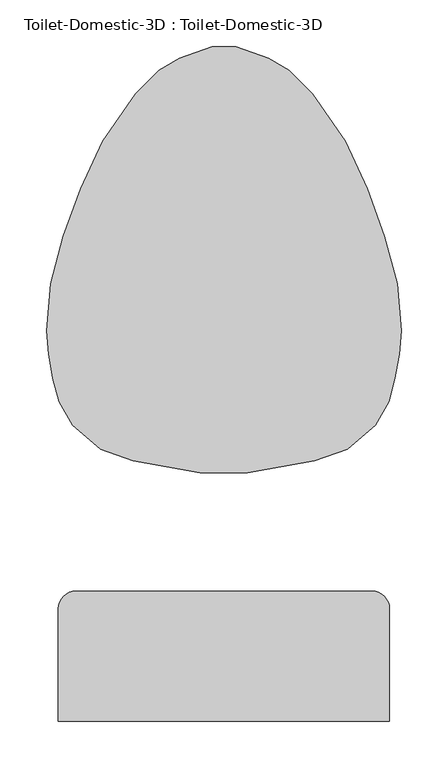
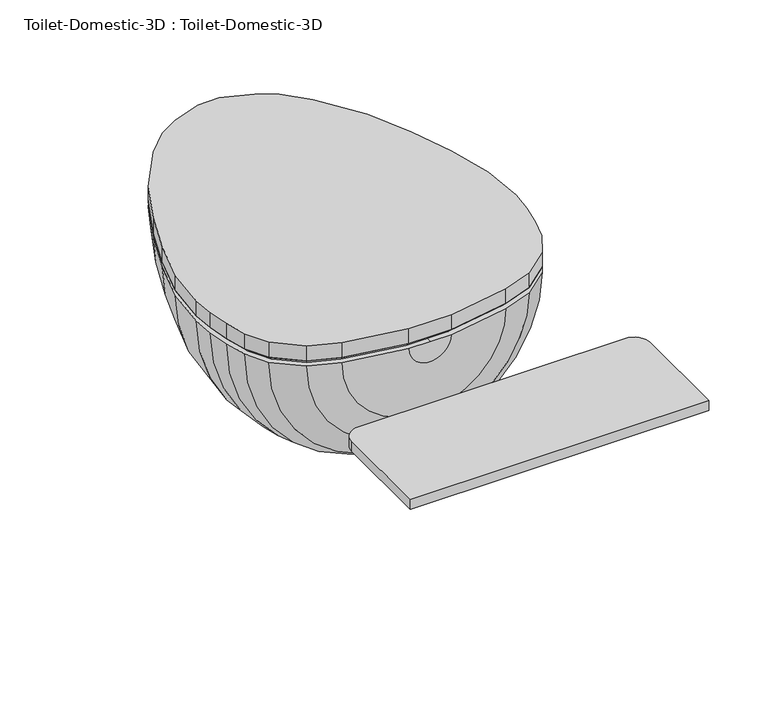
"""IFC4 building model written with IfcOpenShell, lengths in millimetres: flow terminal geometry, Toilet-Domestic-3D : Toilet-Domestic-3D."""

import ifcopenshell
import ifcopenshell.guid

model = None  # the IFC model being written
_history = None  # IfcOwnerHistory: only IFC2X3 demands one
_inside = {}  # id of a spatial element -> (the spatial element, [elements in it])
_under = {}  # id of a project, library or spatial element -> (it, [spatial elements below it])
_declared = {}  # id of a project -> (the project, [libraries it declares])
_typed = {}  # id of a type object -> (the type object, [elements of that type])
_made_of = {}  # id of a material, layer set ... -> (it, [elements and type objects made of it])


def new_model(schema):
    """Start an empty IFC model of exactly this schema.

    Asked for "IFC4X3", IfcOpenShell would pick the latest addendum, in which some entities
    have other attributes; the version numbers below select the first issue.
    IFC2X3 requires an IfcOwnerHistory on every rooted entity: one is made here for all.
    """
    global model, _history
    if schema == "IFC4X3":
        model = ifcopenshell.file(schema_version=(4, 3, 0, 0))
    else:
        model = ifcopenshell.file(schema=schema)
    _inside.clear()
    _under.clear()
    _declared.clear()
    _typed.clear()
    _made_of.clear()
    _history = None
    if model.schema == "IFC2X3":
        org = make("IfcOrganization", Name="unknown")
        user = make(
            "IfcPersonAndOrganization",
            ThePerson=make("IfcPerson", FamilyName="unknown"),
            TheOrganization=org,
        )
        app = make(
            "IfcApplication",
            ApplicationDeveloper=org,
            Version="unknown",
            ApplicationFullName="unknown",
            ApplicationIdentifier="unknown",
        )
        _history = make(
            "IfcOwnerHistory",
            OwningUser=user,
            OwningApplication=app,
            ChangeAction="ADDED",
            CreationDate=0,
        )
    return model


def make(cls, **values):
    """One entity of the class cls with the attributes given. An attribute that is None is left unset."""
    return model.create_entity(
        cls, **{name: value for name, value in values.items() if value is not None}
    )


def rooted(cls, **values):
    """An entity with a GlobalId (a new one), such as an element, a storey or a relation."""
    return make(cls, GlobalId=ifcopenshell.guid.new(), OwnerHistory=_history, **values)


def si_unit(unit_type, name, prefix=None):
    """IfcSIUnit, for example si_unit("LENGTHUNIT", "METRE", prefix="MILLI")."""
    return make("IfcSIUnit", UnitType=unit_type, Prefix=prefix, Name=name)


def assignment(units):
    """IfcUnitAssignment: the units of a project."""
    return None if units is None else make("IfcUnitAssignment", Units=units)


def point(xyz):
    """IfcCartesianPoint."""
    return None if xyz is None else make("IfcCartesianPoint", Coordinates=xyz)


def direction(xyz):
    """IfcDirection."""
    return None if xyz is None else make("IfcDirection", DirectionRatios=xyz)


def frame(location, z_axis=None, x_axis=None):
    """IfcAxis2Placement3D, a coordinate frame: its origin and axes. An axis left out is left unset."""
    return make(
        "IfcAxis2Placement3D",
        Location=point(location),
        Axis=direction(z_axis),
        RefDirection=direction(x_axis),
    )


def frame_2d(location, x_axis=None):
    """IfcAxis2Placement2D, a coordinate frame in the plane: its origin and x axis."""
    return make(
        "IfcAxis2Placement2D", Location=point(location), RefDirection=direction(x_axis)
    )


def origin():
    """The frame at (0, 0, 0) with its axes left unset."""
    return frame((0.0, 0.0, 0.0))


def place(relative_to, where):
    """IfcLocalPlacement: puts the frame where relative to a parent placement (None: the world)."""
    return make(
        "IfcLocalPlacement", PlacementRelTo=relative_to, RelativePlacement=where
    )


def context(
    kind, dimensions, precision=None, world=None, true_north=None, identifier=None
):
    """IfcGeometricRepresentationContext, for example the 3D "Model" context."""
    return make(
        "IfcGeometricRepresentationContext",
        ContextIdentifier=identifier,
        ContextType=kind,
        CoordinateSpaceDimension=dimensions,
        Precision=precision,
        WorldCoordinateSystem=world,
        TrueNorth=true_north,
    )


def project(units=None, contexts=None):
    """IfcProject with its units and contexts."""
    return rooted(
        "IfcProject",
        Name="project",
        RepresentationContexts=contexts,
        UnitsInContext=assignment(units),
    )


def spatial(cls, under=None, at=None, **own):
    """A site, building, storey or space (cls), placed at a placement, below another one or the project."""
    s = rooted(cls, ObjectPlacement=at, **own)
    if under is not None:
        _under.setdefault(under.id(), (under, []))[1].append(s)
    return s


def polyline(points):
    """IfcPolyline through the points."""
    return make("IfcPolyline", Points=[point(p) for p in points])


def circle_curve(where, radius):
    """IfcCircle in the frame where."""
    return make("IfcCircle", Position=where, Radius=radius)


def trimmed(basis, trim1, trim2, sense, master):
    """IfcTrimmedCurve: the piece of a basis curve between two trims."""
    return make(
        "IfcTrimmedCurve",
        BasisCurve=basis,
        Trim1=trim1,
        Trim2=trim2,
        SenseAgreement=sense,
        MasterRepresentation=master,
    )


def segment(curve, same_sense, transition):
    """IfcCompositeCurveSegment."""
    return make(
        "IfcCompositeCurveSegment",
        Transition=transition,
        SameSense=same_sense,
        ParentCurve=curve,
    )


def composite_curve(segments, self_intersect=None):
    """IfcCompositeCurve: segments joined end to end."""
    return make("IfcCompositeCurve", Segments=segments, SelfIntersect=self_intersect)


def outline(outer, holes=None, kind="AREA"):
    """IfcArbitraryClosedProfileDef: a profile drawn as a closed curve; with holes, ...WithVoids."""
    if holes is None:
        return make("IfcArbitraryClosedProfileDef", ProfileType=kind, OuterCurve=outer)
    return make(
        "IfcArbitraryProfileDefWithVoids",
        ProfileType=kind,
        OuterCurve=outer,
        InnerCurves=holes,
    )


def extrude(swept, where, along, depth):
    """IfcExtrudedAreaSolid: the profile swept, set in the frame where, extruded along a direction by depth."""
    return make(
        "IfcExtrudedAreaSolid",
        SweptArea=swept,
        Position=where,
        ExtrudedDirection=direction(along),
        Depth=depth,
    )


def faces_of(points, faces, orient=None, outer=None):
    """IfcFace entities. A face is a list of loops; a loop is a list of indices into points, from 0.

    orient and outer hold one flag for each loop. By default every Orientation is true, the
    first loop of a face is its IfcFaceOuterBound and the others are IfcFaceBound.
    """
    made = []
    for i, loops in enumerate(faces):
        bounds = []
        for j, loop in enumerate(loops):
            is_outer = j == 0 if outer is None else outer[i][j]
            bounds.append(
                make(
                    "IfcFaceOuterBound" if is_outer else "IfcFaceBound",
                    Bound=make("IfcPolyLoop", Polygon=[points[k] for k in loop]),
                    Orientation=True if orient is None else orient[i][j],
                )
            )
        made.append(make("IfcFace", Bounds=bounds))
    return made


def faceted_brep(points, faces, orient=None, outer=None, voids=None):
    """IfcFacetedBrep: a solid bounded by flat faces; with voids (closed shells), ...WithVoids."""
    shared = [point(p) for p in points]
    hull = make("IfcClosedShell", CfsFaces=faces_of(shared, faces, orient, outer))
    if voids is None:
        return make("IfcFacetedBrep", Outer=hull)
    return make(
        "IfcFacetedBrepWithVoids",
        Outer=hull,
        Voids=[
            make(cls, CfsFaces=faces_of(shared, fs, o, b)) for cls, fs, o, b in voids
        ],
    )


def shape(context_of_items, identifier, shape_type, items):
    """IfcShapeRepresentation: the items that make up one representation, for example the "Body"."""
    return make(
        "IfcShapeRepresentation",
        ContextOfItems=context_of_items,
        RepresentationIdentifier=identifier,
        RepresentationType=shape_type,
        Items=items,
    )


def source(mapping_origin, context_of_items, identifier, shape_type, items):
    """IfcRepresentationMap: a shape defined once, which mapped items show again and again."""
    return make(
        "IfcRepresentationMap",
        MappingOrigin=mapping_origin,
        MappedRepresentation=shape(context_of_items, identifier, shape_type, items),
    )


def transform(
    local_origin,
    x_axis=None,
    y_axis=None,
    z_axis=None,
    scale=None,
    scale2=None,
    scale3=None,
    uniform=True,
):
    """IfcCartesianTransformationOperator3D, or its non-uniform kind. x_axis, y_axis, z_axis: its Axis1, 2, 3."""
    if uniform:
        return make(
            "IfcCartesianTransformationOperator3D",
            Axis1=direction(x_axis),
            Axis2=direction(y_axis),
            LocalOrigin=point(local_origin),
            Scale=scale,
            Axis3=direction(z_axis),
        )
    return make(
        "IfcCartesianTransformationOperator3DnonUniform",
        Axis1=direction(x_axis),
        Axis2=direction(y_axis),
        LocalOrigin=point(local_origin),
        Scale=scale,
        Axis3=direction(z_axis),
        Scale2=scale2,
        Scale3=scale3,
    )


def mapped(mapping_source, mapping_target):
    """IfcMappedItem: shows the shape of a source again, moved by a transform."""
    return make(
        "IfcMappedItem", MappingSource=mapping_source, MappingTarget=mapping_target
    )


def made_of(thing, what):
    """Note that an element or type object is made of a material, layer set ...; save() writes the relation."""
    if what is not None:
        _made_of.setdefault(what.id(), (what, []))[1].append(thing)
    return thing


def element(
    cls,
    number,
    at=None,
    inside=None,
    cuts=None,
    type_object=None,
    material=None,
    context=None,
    identifier="Body",
    shape_type=None,
    held_by="IfcProductDefinitionShape",
    body=None,
    shapes=None,
    **own,
):
    """One element of the class cls, such as IfcWall. Its Tag is "e" and its number.

    at: its placement. inside: the storey or other place that contains it. cuts: it is an
    opening in that element (IfcRelVoidsElement). A single representation is given by context,
    identifier, shape_type and body (its items); several are given by shapes. held_by: the class
    of the entity that holds the representations. save() writes the other relations.
    """
    e = rooted(cls, Tag="e%d" % number, ObjectPlacement=at, **own)
    if body is not None:
        shapes = [shape(context, identifier, shape_type, body)]
    if shapes is not None:
        e.Representation = make(held_by, Representations=shapes)
    if inside is not None:
        _inside.setdefault(inside.id(), (inside, []))[1].append(e)
    if cuts is not None:
        rooted(
            "IfcRelVoidsElement", RelatingBuildingElement=cuts, RelatedOpeningElement=e
        )
    if type_object is not None:
        _typed.setdefault(type_object.id(), (type_object, []))[1].append(e)
    return made_of(e, material)


def aggregate(whole, parts):
    """IfcRelAggregates: a whole, such as a stair, and the parts it consists of."""
    return rooted("IfcRelAggregates", RelatingObject=whole, RelatedObjects=parts)


def save(model, path):
    """Write the relations noted so far, then the file.

    IfcRelAggregates (storeys below a building ...), IfcRelContainedInSpatialStructure (elements
    in a storey), IfcRelDefinesByType, IfcRelAssociatesMaterial and IfcRelDeclares: one each for
    every whole, place, type object, material and project.
    """
    for whole, parts in _under.values():
        aggregate(whole, parts)
    for where, things in _inside.values():
        rooted(
            "IfcRelContainedInSpatialStructure",
            RelatedElements=things,
            RelatingStructure=where,
        )
    for kind, things in _typed.values():
        rooted("IfcRelDefinesByType", RelatedObjects=things, RelatingType=kind)
    for what, things in _made_of.values():
        rooted("IfcRelAssociatesMaterial", RelatedObjects=things, RelatingMaterial=what)
    for by, libraries in _declared.values():
        rooted("IfcRelDeclares", RelatingContext=by, RelatedDefinitions=libraries)
    model.write(path)


def plane_surface(at):
    """IfcPlane: the flat surface through the origin of the frame at, square to its z axis."""
    return make("IfcPlane", Position=at)


def revolved_surface(curve, axis_point, axis_direction):
    """IfcSurfaceOfRevolution: the curve turned about the line through axis_point along axis_direction."""
    return make(
        "IfcSurfaceOfRevolution",
        SweptCurve=make("IfcArbitraryOpenProfileDef", ProfileType="CURVE", Curve=curve),
        AxisPosition=make("IfcAxis1Placement", Location=point(axis_point), Axis=direction(axis_direction)),
    )


def advanced_brep(points, edges, surfaces, faces):
    """IfcAdvancedBrep: a solid bounded by faces that lie on surfaces and meet in shared edges.

    An edge is (start, end): straight between two places in points (the first is 0);
    or (start, end, curve); or (start, end, curve, False) where it runs against its curve.
    A face is (place in surfaces, loops), or (place, loops, False) where it looks against
    its surface's normal. A loop lists edges by number (the first is 1), with a minus sign
    where the edge is run from its end to its start. The first loop is the outer one.
    """
    corners = [point(p) for p in points]
    vertices = [make("IfcVertexPoint", VertexGeometry=c) for c in corners]
    made = []
    for start, end, *more in edges:
        made.append(
            make(
                "IfcEdgeCurve",
                EdgeStart=vertices[start],
                EdgeEnd=vertices[end],
                EdgeGeometry=more[0] if more else make("IfcPolyline", Points=[corners[start], corners[end]]),
                SameSense=more[1] if len(more) > 1 else True,
            )
        )
    hull = []
    for where, loops, *sense in faces:
        bounds = []
        for j, loop in enumerate(loops):
            ring = [make("IfcOrientedEdge", EdgeElement=made[abs(k) - 1], Orientation=k > 0) for k in loop]
            bounds.append(
                make(
                    "IfcFaceOuterBound" if j == 0 else "IfcFaceBound",
                    Bound=make("IfcEdgeLoop", EdgeList=ring),
                    Orientation=True,
                )
            )
        hull.append(make("IfcAdvancedFace", Bounds=bounds, FaceSurface=surfaces[where], SameSense=sense[0] if sense else True))
    return make("IfcAdvancedBrep", Outer=make("IfcClosedShell", CfsFaces=hull))


def toilet_domestic_3d_toilet_domestic_3d_5530cc89(model_context):
    return source(origin(), model_context, "Body", "SolidModel", [
        advanced_brep(
        [(-25.4, -152.4, 361.95), (0.0, -152.4, 361.95), (0.0, -133.6394123, 361.95), (-22.0920022, -133.6394123, 361.95), (-94.1172813, -120.9394123, 361.95), (-121.9980886, -110.7916284, 361.95), (-146.1085923, -90.5605136, 361.95), (-159.5484355, -68.2281551, 361.95), (-165.101298, -47.5045901, 361.95), (-169.3087351, -23.6430284, 361.95), (-171.5645445, 2.1409906, 361.95), (-167.7238545, 46.0402777, 361.95), (-154.575847, 95.1093097, 361.95), (-136.654021, 144.3491221, 361.95), (-114.0255101, 192.8761202, 361.95), (-79.2146703, 243.0564036, 361.95), (-58.4178985, 263.8531754, 361.95), (-39.5113323, 274.7688865, 361.95), (-12.5224565, 284.592034, 361.95), (0.0, 284.592034, 361.95), (0.0, 304.8, 361.95), (-12.7, 304.8, 361.95), (-47.5929632, 292.1, 361.95), (-69.5900085, 279.4, 361.95), (-94.9900085, 254.0, 361.95), (-130.2307553, 203.2, 361.95), (-153.9191843, 152.4, 361.95), (-172.4088722, 101.6, 361.95), (-186.0724883, 50.6066907, 361.95), (-190.5, 0.0, 361.95), (-188.2862441, -25.3033453, 361.95), (-183.790496, -50.8, 361.95), (-176.9845865, -76.2, 361.95), (-162.5887836, -101.6, 361.95), (-132.3182423, -127.0, 361.95), (-97.4252791, -139.7, 361.95), (25.4, -152.4, 361.95), (97.4252791, -139.7, 361.95), (132.3182423, -127.0, 361.95), (162.5887836, -101.6, 361.95), (176.9845865, -76.2, 361.95), (183.790496, -50.8, 361.95), (188.2862441, -25.3033453, 361.95), (190.5, 0.0, 361.95), (186.0724883, 50.6066907, 361.95), (172.4088722, 101.6, 361.95), (153.9191843, 152.4, 361.95), (130.2307553, 203.2, 361.95), (94.9900085, 254.0, 361.95), (69.5900085, 279.4, 361.95), (47.5929632, 292.1, 361.95), (12.7, 304.8, 361.95), (12.5224565, 284.592034, 361.95), (39.5113323, 274.7688865, 361.95), (58.4178985, 263.8531754, 361.95), (79.2146703, 243.0564036, 361.95), (114.0255101, 192.8761202, 361.95), (136.654021, 144.3491221, 361.95), (154.575847, 95.1093097, 361.95), (167.7238545, 46.0402777, 361.95), (171.5645445, 2.1409906, 361.95), (169.3087351, -23.6430284, 361.95), (165.101298, -47.5045901, 361.95), (159.5484355, -68.2281551, 361.95), (146.1085923, -90.5605136, 361.95), (121.9980886, -110.7916284, 361.95), (94.1172813, -120.9394123, 361.95), (22.0920022, -133.6394123, 361.95)],
        [
            (0, 1),
            (1, 2),
            (2, 3),
            (3, 4),
            (4, 5),
            (5, 6),
            (6, 7),
            (7, 8),
            (8, 9),
            (9, 10),
            (10, 11),
            (11, 12),
            (12, 13),
            (13, 14),
            (14, 15),
            (15, 16),
            (16, 17),
            (17, 18),
            (18, 19),
            (19, 20),
            (20, 21),
            (21, 22),
            (22, 23),
            (23, 24),
            (24, 25),
            (25, 26),
            (26, 27),
            (27, 28),
            (28, 29),
            (29, 30),
            (30, 31),
            (31, 32),
            (32, 33),
            (33, 34),
            (34, 35),
            (35, 0),
            (36, 37),
            (37, 38),
            (38, 39),
            (39, 40),
            (40, 41),
            (41, 42),
            (42, 43),
            (43, 44),
            (44, 45),
            (45, 46),
            (46, 47),
            (47, 48),
            (48, 49),
            (49, 50),
            (50, 51),
            (51, 20),
            (19, 52),
            (52, 53),
            (53, 54),
            (54, 55),
            (55, 56),
            (56, 57),
            (57, 58),
            (58, 59),
            (59, 60),
            (60, 61),
            (61, 62),
            (62, 63),
            (63, 64),
            (64, 65),
            (65, 66),
            (66, 67),
            (67, 2),
            (1, 36),
            (36, 0, circle_curve(frame((0.0, -152.4, 361.95), z_axis=(0.0, 1.0, 0.0), x_axis=(-1.0, 0.0, 0.0)), 25.4)),
            (35, 37, circle_curve(frame((0.0, -139.7, 361.95), z_axis=(0.0, -1.0, 0.0), x_axis=(-1.0, 0.0, 0.0)), 97.4252791)),
            (34, 38, circle_curve(frame((0.0, -127.0, 361.95), z_axis=(0.0, -1.0, 0.0), x_axis=(-1.0, 0.0, 0.0)), 132.3182423)),
            (33, 39, circle_curve(frame((0.0, -101.6, 361.95), z_axis=(0.0, -1.0, 0.0), x_axis=(-1.0, 0.0, 0.0)), 162.5887836)),
            (32, 40, circle_curve(frame((0.0, -76.2, 361.95), z_axis=(0.0, -1.0, 0.0), x_axis=(-1.0, 0.0, 0.0)), 176.9845865)),
            (31, 41, circle_curve(frame((0.0, -50.8, 361.95), z_axis=(0.0, -1.0, 0.0), x_axis=(-1.0, 0.0, 0.0)), 183.790496)),
            (30, 42, circle_curve(frame((0.0, -25.3033453, 361.95), z_axis=(0.0, -1.0, 0.0), x_axis=(-1.0, 0.0, 0.0)), 188.2862441)),
            (29, 43, circle_curve(frame((0.0, 0.0, 361.95), z_axis=(0.0, -1.0, 0.0), x_axis=(-1.0, 0.0, 0.0)), 190.5)),
            (28, 44, circle_curve(frame((0.0, 50.6066907, 361.95), z_axis=(0.0, -1.0, 0.0), x_axis=(-1.0, 0.0, 0.0)), 186.0724883)),
            (27, 45, circle_curve(frame((0.0, 101.6, 361.95), z_axis=(0.0, -1.0, 0.0), x_axis=(-1.0, 0.0, 0.0)), 172.4088722)),
            (26, 46, circle_curve(frame((0.0, 152.4, 361.95), z_axis=(0.0, -1.0, 0.0), x_axis=(-1.0, 0.0, 0.0)), 153.9191843)),
            (25, 47, circle_curve(frame((0.0, 203.2, 361.95), z_axis=(0.0, -1.0, 0.0), x_axis=(-1.0, 0.0, 0.0)), 130.2307553)),
            (24, 48, circle_curve(frame((0.0, 254.0, 361.95), z_axis=(0.0, -1.0, 0.0), x_axis=(-1.0, 0.0, 0.0)), 94.9900085)),
            (23, 49, circle_curve(frame((0.0, 279.4, 361.95), z_axis=(0.0, -1.0, 0.0), x_axis=(-1.0, 0.0, 0.0)), 69.5900085)),
            (22, 50, circle_curve(frame((0.0, 292.1, 361.95), z_axis=(0.0, -1.0, 0.0), x_axis=(-1.0, 0.0, 0.0)), 47.5929632)),
            (21, 51, circle_curve(frame((0.0, 304.8, 361.95), z_axis=(0.0, -1.0, 0.0), x_axis=(-1.0, 0.0, 0.0)), 12.7)),
            (18, 52, circle_curve(frame((0.0, 284.592034, 361.95), z_axis=(0.0, -1.0, 0.0), x_axis=(-1.0, 0.0, 0.0)), 12.5224565)),
            (17, 53, circle_curve(frame((0.0, 274.7688865, 361.95), z_axis=(0.0, -1.0, 0.0), x_axis=(-1.0, 0.0, 0.0)), 39.5113323)),
            (16, 54, circle_curve(frame((0.0, 263.8531754, 361.95), z_axis=(0.0, -1.0, 0.0), x_axis=(-1.0, 0.0, 0.0)), 58.4178985)),
            (15, 55, circle_curve(frame((0.0, 243.0564036, 361.95), z_axis=(0.0, -1.0, 0.0), x_axis=(-1.0, 0.0, 0.0)), 79.2146703)),
            (14, 56, circle_curve(frame((0.0, 192.8761202, 361.95), z_axis=(0.0, -1.0, 0.0), x_axis=(-1.0, 0.0, 0.0)), 114.0255101)),
            (13, 57, circle_curve(frame((0.0, 144.3491221, 361.95), z_axis=(0.0, -1.0, 0.0), x_axis=(-1.0, 0.0, 0.0)), 136.654021)),
            (12, 58, circle_curve(frame((0.0, 95.1093097, 361.95), z_axis=(0.0, -1.0, 0.0), x_axis=(-1.0, 0.0, 0.0)), 154.575847)),
            (11, 59, circle_curve(frame((0.0, 46.0402777, 361.95), z_axis=(0.0, -1.0, 0.0), x_axis=(-1.0, 0.0, 0.0)), 167.7238545)),
            (10, 60, circle_curve(frame((0.0, 2.1409906, 361.95), z_axis=(0.0, -1.0, 0.0), x_axis=(-1.0, 0.0, 0.0)), 171.5645445)),
            (9, 61, circle_curve(frame((0.0, -23.6430284, 361.95), z_axis=(0.0, -1.0, 0.0), x_axis=(-1.0, 0.0, 0.0)), 169.3087351)),
            (8, 62, circle_curve(frame((0.0, -47.5045901, 361.95), z_axis=(0.0, -1.0, 0.0), x_axis=(-1.0, 0.0, 0.0)), 165.101298)),
            (7, 63, circle_curve(frame((0.0, -68.2281551, 361.95), z_axis=(0.0, -1.0, 0.0), x_axis=(-1.0, 0.0, 0.0)), 159.5484355)),
            (6, 64, circle_curve(frame((0.0, -90.5605136, 361.95), z_axis=(0.0, -1.0, 0.0), x_axis=(-1.0, 0.0, 0.0)), 146.1085923)),
            (5, 65, circle_curve(frame((0.0, -110.7916284, 361.95), z_axis=(0.0, -1.0, 0.0), x_axis=(-1.0, 0.0, 0.0)), 121.9980886)),
            (4, 66, circle_curve(frame((0.0, -120.9394123, 361.95), z_axis=(0.0, -1.0, 0.0), x_axis=(-1.0, 0.0, 0.0)), 94.1172813)),
            (3, 67, circle_curve(frame((0.0, -133.6394123, 361.95), z_axis=(0.0, -1.0, 0.0), x_axis=(-1.0, 0.0, 0.0)), 22.0920022)),
        ],
        [
            plane_surface(frame((0.0, -175.1599017, 361.95), z_axis=(0.0, 0.0, 1.0), x_axis=(-1.0, 0.0, 0.0))),
            plane_surface(frame((0.0, -175.1599017, 361.95), z_axis=(0.0, 0.0, 1.0), x_axis=(1.0, 0.0, 0.0))),
            revolved_surface(polyline([(-25.4, -152.4, 361.95), (-97.4252791, -139.7, 361.95)]), (0.0, -175.1599017, 361.95), (0.0, 1.0, 0.0)),
            revolved_surface(polyline([(-97.4252791, -139.7, 361.95), (-132.3182423, -127.0, 361.95)]), (0.0, -175.1599017, 361.95), (0.0, 1.0, 0.0)),
            revolved_surface(polyline([(-132.3182423, -127.0, 361.95), (-162.5887836, -101.6, 361.95)]), (0.0, -175.1599017, 361.95), (0.0, 1.0, 0.0)),
            revolved_surface(polyline([(-162.5887836, -101.6, 361.95), (-176.9845865, -76.2, 361.95)]), (0.0, -175.1599017, 361.95), (0.0, 1.0, 0.0)),
            revolved_surface(polyline([(-176.9845865, -76.2, 361.95), (-183.790496, -50.8, 361.95)]), (0.0, -175.1599017, 361.95), (0.0, 1.0, 0.0)),
            revolved_surface(polyline([(-183.790496, -50.8, 361.95), (-188.2862441, -25.3033453, 361.95)]), (0.0, -175.1599017, 361.95), (0.0, 1.0, 0.0)),
            revolved_surface(polyline([(-188.2862441, -25.3033453, 361.95), (-190.5, 0.0, 361.95)]), (0.0, -175.1599017, 361.95), (0.0, 1.0, 0.0)),
            revolved_surface(polyline([(-190.5, 0.0, 361.95), (-186.0724883, 50.6066907, 361.95)]), (0.0, -175.1599017, 361.95), (0.0, 1.0, 0.0)),
            revolved_surface(polyline([(-186.0724883, 50.6066907, 361.95), (-172.4088722, 101.6, 361.95)]), (0.0, -175.1599017, 361.95), (0.0, 1.0, 0.0)),
            revolved_surface(polyline([(-172.4088722, 101.6, 361.95), (-153.9191843, 152.4, 361.95)]), (0.0, -175.1599017, 361.95), (0.0, 1.0, 0.0)),
            revolved_surface(polyline([(-153.9191843, 152.4, 361.95), (-130.2307553, 203.2, 361.95)]), (0.0, -175.1599017, 361.95), (0.0, 1.0, 0.0)),
            revolved_surface(polyline([(-130.2307553, 203.2, 361.95), (-94.9900085, 254.0, 361.95)]), (0.0, -175.1599017, 361.95), (0.0, 1.0, 0.0)),
            revolved_surface(polyline([(-94.9900085, 254.0, 361.95), (-69.5900085, 279.4, 361.95)]), (0.0, -175.1599017, 361.95), (0.0, 1.0, 0.0)),
            revolved_surface(polyline([(-69.5900085, 279.4, 361.95), (-47.5929632, 292.1, 361.95)]), (0.0, -175.1599017, 361.95), (0.0, 1.0, 0.0)),
            revolved_surface(polyline([(-47.5929632, 292.1, 361.95), (-12.7, 304.8, 361.95)]), (0.0, -175.1599017, 361.95), (0.0, 1.0, 0.0)),
            plane_surface(frame((0.0, 304.8, 361.95), z_axis=(0.0, 1.0, 0.0), x_axis=(-1.0, 0.0, 0.0))),
            plane_surface(frame((0.0, 284.592034, 361.95), z_axis=(0.0, -1.0, 0.0), x_axis=(-1.0, 0.0, 0.0))),
            revolved_surface(polyline([(-12.5224565, 284.592034, 361.95), (-39.5113323, 274.7688865, 361.95)]), (0.0, -175.1599017, 361.95), (0.0, 1.0, 0.0)),
            revolved_surface(polyline([(-39.5113323, 274.7688865, 361.95), (-58.4178985, 263.8531754, 361.95)]), (0.0, -175.1599017, 361.95), (0.0, 1.0, 0.0)),
            revolved_surface(polyline([(-58.4178985, 263.8531754, 361.95), (-79.2146703, 243.0564036, 361.95)]), (0.0, -175.1599017, 361.95), (0.0, 1.0, 0.0)),
            revolved_surface(polyline([(-79.2146703, 243.0564036, 361.95), (-114.0255101, 192.8761202, 361.95)]), (0.0, -175.1599017, 361.95), (0.0, 1.0, 0.0)),
            revolved_surface(polyline([(-114.0255101, 192.8761202, 361.95), (-136.654021, 144.3491221, 361.95)]), (0.0, -175.1599017, 361.95), (0.0, 1.0, 0.0)),
            revolved_surface(polyline([(-136.654021, 144.3491221, 361.95), (-154.575847, 95.1093097, 361.95)]), (0.0, -175.1599017, 361.95), (0.0, 1.0, 0.0)),
            revolved_surface(polyline([(-154.575847, 95.1093097, 361.95), (-167.7238545, 46.0402777, 361.95)]), (0.0, -175.1599017, 361.95), (0.0, 1.0, 0.0)),
            revolved_surface(polyline([(-167.7238545, 46.0402777, 361.95), (-171.5645445, 2.1409906, 361.95)]), (0.0, -175.1599017, 361.95), (0.0, 1.0, 0.0)),
            revolved_surface(polyline([(-171.5645445, 2.1409906, 361.95), (-169.3087351, -23.6430284, 361.95)]), (0.0, -175.1599017, 361.95), (0.0, 1.0, 0.0)),
            revolved_surface(polyline([(-169.3087351, -23.6430284, 361.95), (-165.101298, -47.5045901, 361.95)]), (0.0, -175.1599017, 361.95), (0.0, 1.0, 0.0)),
            revolved_surface(polyline([(-165.101298, -47.5045901, 361.95), (-159.5484355, -68.2281551, 361.95)]), (0.0, -175.1599017, 361.95), (0.0, 1.0, 0.0)),
            revolved_surface(polyline([(-159.5484355, -68.2281551, 361.95), (-146.1085923, -90.5605136, 361.95)]), (0.0, -175.1599017, 361.95), (0.0, 1.0, 0.0)),
            revolved_surface(polyline([(-146.1085923, -90.5605136, 361.95), (-121.9980886, -110.7916284, 361.95)]), (0.0, -175.1599017, 361.95), (0.0, 1.0, 0.0)),
            revolved_surface(polyline([(-121.9980886, -110.7916284, 361.95), (-94.1172813, -120.9394123, 361.95)]), (0.0, -175.1599017, 361.95), (0.0, 1.0, 0.0)),
            revolved_surface(polyline([(-94.1172813, -120.9394123, 361.95), (-22.0920022, -133.6394123, 361.95)]), (0.0, -175.1599017, 361.95), (0.0, 1.0, 0.0)),
            plane_surface(frame((0.0, -133.6394123, 361.95), z_axis=(0.0, 1.0, 0.0), x_axis=(-1.0, 0.0, 0.0))),
            plane_surface(frame((0.0, -152.4, 361.95), z_axis=(0.0, -1.0, 0.0), x_axis=(-1.0, 0.0, 0.0))),
        ],
        [
            (0, [[1, 2, 3, 4, 5, 6, 7, 8, 9, 10, 11, 12, 13, 14, 15, 16, 17, 18, 19, 20, 21, 22, 23, 24, 25, 26, 27, 28, 29, 30, 31, 32, 33, 34, 35, 36]]),
            (1, [[37, 38, 39, 40, 41, 42, 43, 44, 45, 46, 47, 48, 49, 50, 51, 52, -20, 53, 54, 55, 56, 57, 58, 59, 60, 61, 62, 63, 64, 65, 66, 67, 68, 69, -2, 70]]),
            (2, [[-37, 71, -36, 72]]),
            (3, [[-38, -72, -35, 73]]),
            (4, [[-39, -73, -34, 74]]),
            (5, [[-40, -74, -33, 75]]),
            (6, [[-41, -75, -32, 76]]),
            (7, [[-42, -76, -31, 77]]),
            (8, [[-43, -77, -30, 78]]),
            (9, [[-44, -78, -29, 79]]),
            (10, [[-45, -79, -28, 80]]),
            (11, [[-46, -80, -27, 81]]),
            (12, [[-47, -81, -26, 82]]),
            (13, [[-48, -82, -25, 83]]),
            (14, [[-49, -83, -24, 84]]),
            (15, [[-50, -84, -23, 85]]),
            (16, [[-51, -85, -22, 86]]),
            (17, [[-52, -86, -21]]),
            (18, [[-53, -19, 87]]),
            (19, [[-54, -87, -18, 88]]),
            (20, [[-55, -88, -17, 89]]),
            (21, [[-56, -89, -16, 90]]),
            (22, [[-57, -90, -15, 91]]),
            (23, [[-58, -91, -14, 92]]),
            (24, [[-59, -92, -13, 93]]),
            (25, [[-60, -93, -12, 94]]),
            (26, [[-61, -94, -11, 95]]),
            (27, [[-62, -95, -10, 96]]),
            (28, [[-63, -96, -9, 97]]),
            (29, [[-64, -97, -8, 98]]),
            (30, [[-65, -98, -7, 99]]),
            (31, [[-66, -99, -6, 100]]),
            (32, [[-67, -100, -5, 101]]),
            (33, [[-68, -101, -4, 102]]),
            (34, [[-69, -102, -3]]),
            (35, [[-70, -1, -71]]),
        ],
    ),
        faceted_brep([(-97.4252791, -139.7, 368.3), (-25.4, -152.4, 368.3), (25.4, -152.4, 368.3), (97.4252791, -139.7, 368.3), (132.3182423, -127.0, 368.3), (162.5887836, -101.6, 368.3), (176.9845865, -76.2, 368.3), (183.790496, -50.8, 368.3), (188.2862441, -25.3033453, 368.3), (190.5, 0.0, 368.3), (186.0724883, 50.6066907, 368.3), (172.4088722, 101.6, 368.3), (153.9191843, 152.4, 368.3), (130.2307553, 203.2, 368.3), (94.9900085, 254.0, 368.3), (69.5900085, 279.4, 368.3), (47.5929632, 292.1, 368.3), (12.7, 304.8, 368.3), (-12.7, 304.8, 368.3), (-47.5929632, 292.1, 368.3), (-69.5900085, 279.4, 368.3), (-94.9900085, 254.0, 368.3), (-130.2307553, 203.2, 368.3), (-153.9191843, 152.4, 368.3), (-172.4088722, 101.6, 368.3), (-186.0724883, 50.6066907, 368.3), (-190.5, 0.0, 368.3), (-188.2862441, -25.3033453, 368.3), (-183.790496, -50.8, 368.3), (-176.9845865, -76.2, 368.3), (-162.5887836, -101.6, 368.3), (-132.3182423, -127.0, 368.3), (-95.7755003, -133.5429415, 361.95), (-129.0942628, -121.4159037, 361.95), (-157.6293435, -97.472128, 361.95), (-171.060664, -73.773864, 361.95), (-177.5851102, -49.4242991, 361.95), (-181.9845715, -24.4737144, 361.95), (-184.125744, 0.0, 361.95), (-179.7950716, 49.4998127, 361.95), (-166.347, 99.688699, 361.95), (-148.0469602, 149.9676451, 361.95), (-124.7045808, 200.0255393, 361.95), (-90.0971582, 249.9125941, 361.95), (-65.691017, 274.3187354, 361.95), (-44.8990862, 286.3229622, 361.95), (-11.5803237, 298.45, 361.95), (11.5803237, 298.45, 361.95), (44.8990862, 286.3229622, 361.95), (65.691017, 274.3187354, 361.95), (90.0971582, 249.9125941, 361.95), (124.7045808, 200.0255393, 361.95), (148.0469602, 149.9676451, 361.95), (166.347, 99.688699, 361.95), (179.7950716, 49.4998127, 361.95), (184.125744, 0.0, 361.95), (181.9845715, -24.4737144, 361.95), (177.5851102, -49.4242991, 361.95), (171.060664, -73.773864, 361.95), (157.6293435, -97.472128, 361.95), (129.0942628, -121.4159037, 361.95), (95.7755003, -133.5429415, 361.95), (24.844447, -146.05, 361.95), (-24.844447, -146.05, 361.95)], [[[0, 1, 2, 3, 4, 5, 6, 7, 8, 9, 10, 11, 12, 13, 14, 15, 16, 17, 18, 19, 20, 21, 22, 23, 24, 25, 26, 27, 28, 29, 30, 31]], [[32, 33, 34, 35, 36, 37, 38, 39, 40, 41, 42, 43, 44, 45, 46, 47, 48, 49, 50, 51, 52, 53, 54, 55, 56, 57, 58, 59, 60, 61, 62, 63]], [[32, 0, 31, 33]], [[33, 31, 30, 34]], [[34, 30, 29, 35]], [[35, 29, 28, 36]], [[36, 28, 27, 37]], [[37, 27, 26, 38]], [[38, 26, 25, 39]], [[39, 25, 24, 40]], [[40, 24, 23, 41]], [[41, 23, 22, 42]], [[42, 22, 21, 43]], [[43, 21, 20, 44]], [[44, 20, 19, 45]], [[45, 19, 18, 46]], [[46, 18, 17, 47]], [[47, 17, 16, 48]], [[48, 16, 15, 49]], [[49, 15, 14, 50]], [[50, 14, 13, 51]], [[51, 13, 12, 52]], [[52, 12, 11, 53]], [[53, 11, 10, 54]], [[54, 10, 9, 55]], [[55, 9, 8, 56]], [[56, 8, 7, 57]], [[57, 7, 6, 58]], [[58, 6, 5, 59]], [[59, 5, 4, 60]], [[60, 4, 3, 61]], [[61, 3, 2, 62]], [[62, 2, 1, 63]], [[63, 1, 0, 32]]]),
        extrude(outline(composite_curve([segment(polyline([(177.8, -419.1), (-177.8, -419.1), (-177.8, -298.45)]), True, "CONTINUOUS"), segment(trimmed(circle_curve(frame_2d((-158.75, -298.45)), 19.05), [point((-177.8, -298.45))], [point((-158.75, -279.4))], False, "CARTESIAN"), True, "CONTINUOUS"), segment(polyline([(-158.75, -279.4), (158.75, -279.4)]), True, "CONTINUOUS"), segment(trimmed(circle_curve(frame_2d((158.75, -298.45)), 19.05), [point((158.75, -279.4))], [point((177.8, -298.45))], False, "CARTESIAN"), True, "CONTINUOUS"), segment(polyline([(177.8, -298.45), (177.8, -419.1)]), True, "CONTINUOUS")], self_intersect=False)), frame((0.0, 0.0, 374.65), z_axis=(0.0, 0.0, 1.0), x_axis=(1.0, 0.0, 0.0)), (0.0, 0.0, 1.0), 12.5681453),
        extrude(outline(polyline([(-162.5887836, -101.6), (-176.9845865, -76.2), (-183.790496, -50.8), (-188.2862441, -25.3033453), (-190.5, 0.0), (-186.0724883, 50.6066907), (-172.4088722, 101.6), (-153.9191843, 152.4), (-130.2307553, 203.2), (-94.9900085, 254.0), (-69.5900085, 279.4), (-47.5929632, 292.1), (-12.7, 304.8), (12.7, 304.8), (47.5929632, 292.1), (69.5900085, 279.4), (94.9900085, 254.0), (130.2307553, 203.2), (153.9191843, 152.4), (172.4088722, 101.6), (186.0724883, 50.6066907), (190.5, 0.0), (188.2862441, -25.3033453), (183.790496, -50.8), (176.9845865, -76.2), (162.5887836, -101.6), (132.3182423, -127.0), (97.4252791, -139.7), (25.4, -152.4), (-25.4, -152.4), (-97.4252791, -139.7), (-132.3182423, -127.0), (-162.5887836, -101.6)])), frame((0.0, 0.0, 368.3), z_axis=(0.0, 0.0, 1.0), x_axis=(1.0, 0.0, 0.0)), (0.0, 0.0, 1.0), 19.05),
    ])


if __name__ == "__main__":
    model = new_model("IFC4")
    model_context = context("Model", 3, world=origin())
    ifc_project = project(units=[si_unit("LENGTHUNIT", "METRE", prefix="MILLI")], contexts=[model_context])
    site = spatial("IfcSite", under=ifc_project)
    building = spatial("IfcBuilding", under=site)
    placement = place(None, origin())
    toilet_domestic_3d_toilet_domestic_3d_shape = toilet_domestic_3d_toilet_domestic_3d_5530cc89(model_context)
    element("IfcFlowTerminal", 1, ObjectType="Toilet-Domestic-3D : Toilet-Domestic-3D", at=placement, inside=building, context=model_context, shape_type="MappedRepresentation", body=[
        mapped(toilet_domestic_3d_toilet_domestic_3d_shape, transform((0.0, 0.0, 0.0), x_axis=(1.0, 0.0, 0.0), y_axis=(0.0, 1.0, 0.0), z_axis=(0.0, 0.0, 1.0))),
    ])
    save(model, "model.ifc")

# Revit data of these elements
# Type "Toilet-Domestic-3D : Toilet-Domestic-3D"
#   Assembly Code = "D2010110"
#   Toilet - Bowl/Basin Material = Porcelain, White
#   Toilet - Seat Material = Laminate, Linen, Matte
#   Default Elevation = 0
# Element 1 (IfcFlowTerminal, "Toilet-Domestic-3D : Toilet-Domestic-3D")
#   Materials on its faces: "Porcelain, White", "Porcelain, Linen", "Laminate, Linen, Matte"
# Materials
#   "Porcelain, White": class "Ceramic", colour RGB 244 244 244, transparency 0, Description = "Porcelain, ivory", Cost = 0
#   "Laminate, Linen, Matte": class "Plastic", colour RGB 249 239 230, transparency 0, Description = "Plastic Laminate - Linen, Matte", Cost = 0
#   "Porcelain, Linen": class "Ceramic", colour RGB 249 239 230, transparency 0, Description = "Porcelain, linen", Cost = 0
